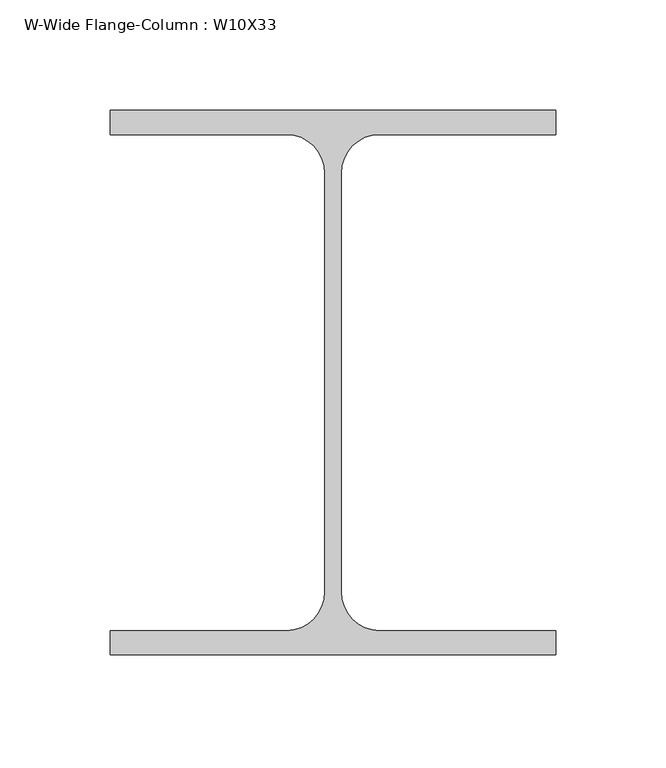
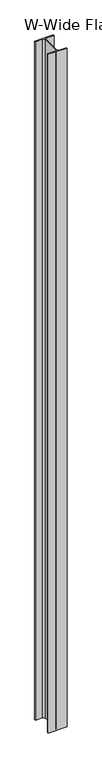
"""IFC4 building model written with IfcOpenShell, lengths in millimetres: column geometry, W-Wide Flange-Column : W10X33."""

from ifc_helpers import new_model, si_unit, point, frame, frame_2d, origin, place, context, project, spatial, polyline, circle_curve, trimmed, segment, composite_curve, outline, extrude, source, transform, mapped, element, save


def w_wide_flange_column_w10x33_52015726(model_context):
    return source(origin(), model_context, "Body", "SweptSolid", [
        extrude(outline(composite_curve([segment(polyline([(101.092, 123.571), (101.092, 112.522), (21.209, 112.522)]), True, "CONTINUOUS"), segment(trimmed(circle_curve(frame_2d((21.209, 94.996)), 17.526), [point((21.209, 112.522))], [point((3.683, 94.996))], True, "CARTESIAN"), True, "CONTINUOUS"), segment(polyline([(3.683, 94.996), (3.683, -94.996)]), True, "CONTINUOUS"), segment(trimmed(circle_curve(frame_2d((21.209, -94.996)), 17.526), [point((3.683, -94.996))], [point((21.209, -112.522))], True, "CARTESIAN"), True, "CONTINUOUS"), segment(polyline([(21.209, -112.522), (101.092, -112.522), (101.092, -123.571), (-101.092, -123.571), (-101.092, -112.522), (-21.209, -112.522)]), True, "CONTINUOUS"), segment(trimmed(circle_curve(frame_2d((-21.209, -94.996)), 17.526), [point((-21.209, -112.522))], [point((-3.683, -94.996))], True, "CARTESIAN"), True, "CONTINUOUS"), segment(polyline([(-3.683, -94.996), (-3.683, 94.996)]), True, "CONTINUOUS"), segment(trimmed(circle_curve(frame_2d((-21.209, 94.996)), 17.526), [point((-3.683, 94.996))], [point((-21.209, 112.522))], True, "CARTESIAN"), True, "CONTINUOUS"), segment(polyline([(-21.209, 112.522), (-101.092, 112.522), (-101.092, 123.571), (101.092, 123.571)]), True, "CONTINUOUS")], self_intersect=False)), frame((0.0, 0.0, 8756.65), z_axis=(0.0, 0.0, 1.0), x_axis=(1.0, 0.0, 0.0)), (0.0, 0.0, 1.0), 7651.75),
    ])


if __name__ == "__main__":
    model = new_model("IFC4")
    model_context = context("Model", 3, world=origin())
    ifc_project = project(units=[si_unit("LENGTHUNIT", "METRE", prefix="MILLI")], contexts=[model_context])
    site = spatial("IfcSite", under=ifc_project)
    building = spatial("IfcBuilding", under=site)
    placement = place(None, origin())
    w_wide_flange_column_w10x33_shape = w_wide_flange_column_w10x33_52015726(model_context)
    element("IfcColumn", 1, ObjectType="W-Wide Flange-Column : W10X33", at=placement, inside=building, context=model_context, shape_type="MappedRepresentation", body=[
        mapped(w_wide_flange_column_w10x33_shape, transform((0.0, 0.0, 0.0), x_axis=(1.0, 0.0, 0.0), y_axis=(0.0, 1.0, 0.0), z_axis=(0.0, 0.0, 1.0))),
    ])
    save(model, "model.ifc")

# Revit data of these elements
# Type "W-Wide Flange-Column : W10X33"
#   Assembly Code = "B10"
#   W = 33
#   bf = 0' - 7.96"
#   d = 0' - 9.73"
#   k = 0' - 1 1/8"
#   kr = 0' - 0.69"
#   tf = 0' - 0.435"
#   tw = 0' - 0.29"
#   A = 0.0674306 SF
#   Structural Material [instance default] = Steel ASTM A992
# Element 1 (IfcColumn, "W-Wide Flange-Column : W10X33")
#   Materials on its faces: "Steel ASTM A992"
# Materials
#   "Steel ASTM A992": class "Metal", colour RGB 199 199 199, transparency 0, Description = "Structural steel 50ksi", Cost = 0
